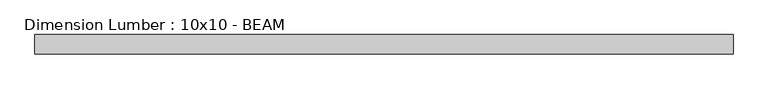
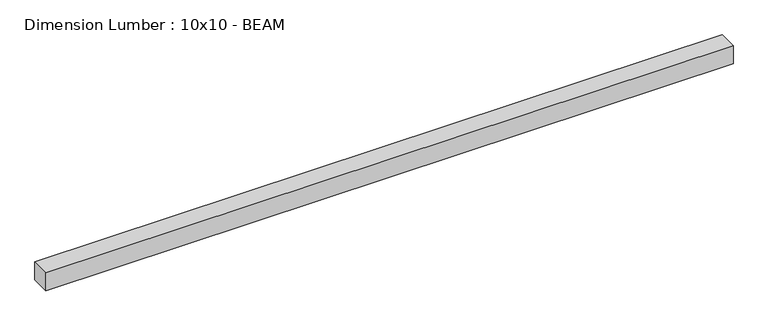
"""IFC4 building model written with IfcOpenShell, lengths in millimetres: beam geometry, Dimension Lumber : 10x10 - BEAM."""

from ifc_helpers import new_model, si_unit, frame, origin, place, context, project, spatial, polyline, outline, extrude, source, transform, mapped, element, save


def dimension_lumber_10x10_beam_e017d86a(model_context):
    return source(origin(), model_context, "Body", "SweptSolid", [
        extrude(outline(polyline([(4267.2, 117.475), (4267.2, -117.475), (-4267.2, -117.475), (-4267.2, 117.475), (4267.2, 117.475)])), frame((0.0, 0.0, -117.475), z_axis=(0.0, 0.0, 1.0), x_axis=(1.0, 0.0, 0.0)), (0.0, 0.0, 1.0), 234.95),
    ])


if __name__ == "__main__":
    model = new_model("IFC4")
    model_context = context("Model", 3, world=origin())
    ifc_project = project(units=[si_unit("LENGTHUNIT", "METRE", prefix="MILLI")], contexts=[model_context])
    site = spatial("IfcSite", under=ifc_project)
    building = spatial("IfcBuilding", under=site)
    placement = place(None, origin())
    dimension_lumber_10x10_beam_shape = dimension_lumber_10x10_beam_e017d86a(model_context)
    element("IfcBeam", 1, ObjectType="Dimension Lumber : 10x10 - BEAM", at=placement, inside=building, context=model_context, shape_type="MappedRepresentation", body=[
        mapped(dimension_lumber_10x10_beam_shape, transform((0.0, 0.0, 0.0), x_axis=(1.0, 0.0, 0.0), y_axis=(0.0, 1.0, 0.0), z_axis=(0.0, 0.0, 1.0))),
    ])
    save(model, "model.ifc")

# Revit data of these elements
# Type "Dimension Lumber : 10x10 - BEAM"
#   Assembly Code = "B10"
#   A = 0.0755556 SF
#   Length [instance default] = 5' - 0"
#   b = 0' - 9 1/4"
#   d = 0' - 9 1/4"
#   Structural Material = (4) CHARRED SISTERED 2X10s AT BEAM
# Element 1 (IfcBeam, "Dimension Lumber : 10x10 - BEAM")
#   Materials on its faces: "(4) CHARRED SISTERED 2X10s AT BEAM"
# Materials
#   "(4) CHARRED SISTERED 2X10s AT BEAM": class "Wood", colour RGB 144 144 144, transparency 0, Description = "Pinus Echinata", Cost = 0
